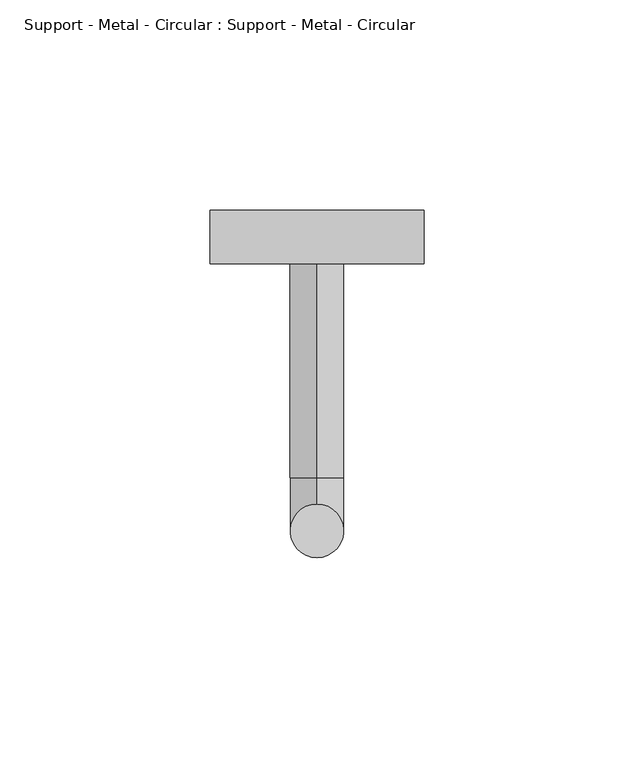
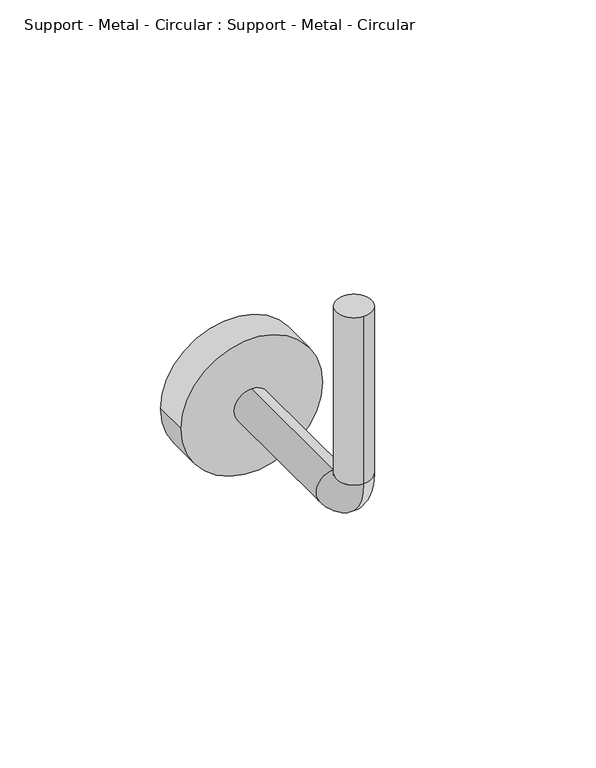
"""IFC4 building model written with IfcOpenShell, lengths in millimetres: proxy geometry, Support - Metal - Circular : Support - Metal - Circular."""

import ifcopenshell
import ifcopenshell.guid

model = None  # the IFC model being written
_history = None  # IfcOwnerHistory: only IFC2X3 demands one
_inside = {}  # id of a spatial element -> (the spatial element, [elements in it])
_under = {}  # id of a project, library or spatial element -> (it, [spatial elements below it])
_declared = {}  # id of a project -> (the project, [libraries it declares])
_typed = {}  # id of a type object -> (the type object, [elements of that type])
_made_of = {}  # id of a material, layer set ... -> (it, [elements and type objects made of it])


def new_model(schema):
    """Start an empty IFC model of exactly this schema.

    Asked for "IFC4X3", IfcOpenShell would pick the latest addendum, in which some entities
    have other attributes; the version numbers below select the first issue.
    IFC2X3 requires an IfcOwnerHistory on every rooted entity: one is made here for all.
    """
    global model, _history
    if schema == "IFC4X3":
        model = ifcopenshell.file(schema_version=(4, 3, 0, 0))
    else:
        model = ifcopenshell.file(schema=schema)
    _inside.clear()
    _under.clear()
    _declared.clear()
    _typed.clear()
    _made_of.clear()
    _history = None
    if model.schema == "IFC2X3":
        org = make("IfcOrganization", Name="unknown")
        user = make(
            "IfcPersonAndOrganization",
            ThePerson=make("IfcPerson", FamilyName="unknown"),
            TheOrganization=org,
        )
        app = make(
            "IfcApplication",
            ApplicationDeveloper=org,
            Version="unknown",
            ApplicationFullName="unknown",
            ApplicationIdentifier="unknown",
        )
        _history = make(
            "IfcOwnerHistory",
            OwningUser=user,
            OwningApplication=app,
            ChangeAction="ADDED",
            CreationDate=0,
        )
    return model


def make(cls, **values):
    """One entity of the class cls with the attributes given. An attribute that is None is left unset."""
    return model.create_entity(
        cls, **{name: value for name, value in values.items() if value is not None}
    )


def rooted(cls, **values):
    """An entity with a GlobalId (a new one), such as an element, a storey or a relation."""
    return make(cls, GlobalId=ifcopenshell.guid.new(), OwnerHistory=_history, **values)


def si_unit(unit_type, name, prefix=None):
    """IfcSIUnit, for example si_unit("LENGTHUNIT", "METRE", prefix="MILLI")."""
    return make("IfcSIUnit", UnitType=unit_type, Prefix=prefix, Name=name)


def assignment(units):
    """IfcUnitAssignment: the units of a project."""
    return None if units is None else make("IfcUnitAssignment", Units=units)


def point(xyz):
    """IfcCartesianPoint."""
    return None if xyz is None else make("IfcCartesianPoint", Coordinates=xyz)


def direction(xyz):
    """IfcDirection."""
    return None if xyz is None else make("IfcDirection", DirectionRatios=xyz)


def frame(location, z_axis=None, x_axis=None):
    """IfcAxis2Placement3D, a coordinate frame: its origin and axes. An axis left out is left unset."""
    return make(
        "IfcAxis2Placement3D",
        Location=point(location),
        Axis=direction(z_axis),
        RefDirection=direction(x_axis),
    )


def frame_2d(location, x_axis=None):
    """IfcAxis2Placement2D, a coordinate frame in the plane: its origin and x axis."""
    return make(
        "IfcAxis2Placement2D", Location=point(location), RefDirection=direction(x_axis)
    )


def origin():
    """The frame at (0, 0, 0) with its axes left unset."""
    return frame((0.0, 0.0, 0.0))


def origin_with_axes():
    """The frame at (0, 0, 0) with the z axis (0, 0, 1) and the x axis (1, 0, 0) written out."""
    return frame((0.0, 0.0, 0.0), z_axis=(0.0, 0.0, 1.0), x_axis=(1.0, 0.0, 0.0))


def place(relative_to, where):
    """IfcLocalPlacement: puts the frame where relative to a parent placement (None: the world)."""
    return make(
        "IfcLocalPlacement", PlacementRelTo=relative_to, RelativePlacement=where
    )


def context(
    kind, dimensions, precision=None, world=None, true_north=None, identifier=None
):
    """IfcGeometricRepresentationContext, for example the 3D "Model" context."""
    return make(
        "IfcGeometricRepresentationContext",
        ContextIdentifier=identifier,
        ContextType=kind,
        CoordinateSpaceDimension=dimensions,
        Precision=precision,
        WorldCoordinateSystem=world,
        TrueNorth=true_north,
    )


def project(units=None, contexts=None):
    """IfcProject with its units and contexts."""
    return rooted(
        "IfcProject",
        Name="project",
        RepresentationContexts=contexts,
        UnitsInContext=assignment(units),
    )


def spatial(cls, under=None, at=None, **own):
    """A site, building, storey or space (cls), placed at a placement, below another one or the project."""
    s = rooted(cls, ObjectPlacement=at, **own)
    if under is not None:
        _under.setdefault(under.id(), (under, []))[1].append(s)
    return s


def circle_curve(where, radius):
    """IfcCircle in the frame where."""
    return make("IfcCircle", Position=where, Radius=radius)


def ellipse_curve(where, semi_axis1, semi_axis2):
    """IfcEllipse in the frame where."""
    return make(
        "IfcEllipse", Position=where, SemiAxis1=semi_axis1, SemiAxis2=semi_axis2
    )


def trimmed(basis, trim1, trim2, sense, master):
    """IfcTrimmedCurve: the piece of a basis curve between two trims."""
    return make(
        "IfcTrimmedCurve",
        BasisCurve=basis,
        Trim1=trim1,
        Trim2=trim2,
        SenseAgreement=sense,
        MasterRepresentation=master,
    )


def segment(curve, same_sense, transition):
    """IfcCompositeCurveSegment."""
    return make(
        "IfcCompositeCurveSegment",
        Transition=transition,
        SameSense=same_sense,
        ParentCurve=curve,
    )


def composite_curve(segments, self_intersect=None):
    """IfcCompositeCurve: segments joined end to end."""
    return make("IfcCompositeCurve", Segments=segments, SelfIntersect=self_intersect)


def outline(outer, holes=None, kind="AREA"):
    """IfcArbitraryClosedProfileDef: a profile drawn as a closed curve; with holes, ...WithVoids."""
    if holes is None:
        return make("IfcArbitraryClosedProfileDef", ProfileType=kind, OuterCurve=outer)
    return make(
        "IfcArbitraryProfileDefWithVoids",
        ProfileType=kind,
        OuterCurve=outer,
        InnerCurves=holes,
    )


def extrude(swept, where, along, depth):
    """IfcExtrudedAreaSolid: the profile swept, set in the frame where, extruded along a direction by depth."""
    return make(
        "IfcExtrudedAreaSolid",
        SweptArea=swept,
        Position=where,
        ExtrudedDirection=direction(along),
        Depth=depth,
    )


def shape(context_of_items, identifier, shape_type, items):
    """IfcShapeRepresentation: the items that make up one representation, for example the "Body"."""
    return make(
        "IfcShapeRepresentation",
        ContextOfItems=context_of_items,
        RepresentationIdentifier=identifier,
        RepresentationType=shape_type,
        Items=items,
    )


def source(mapping_origin, context_of_items, identifier, shape_type, items):
    """IfcRepresentationMap: a shape defined once, which mapped items show again and again."""
    return make(
        "IfcRepresentationMap",
        MappingOrigin=mapping_origin,
        MappedRepresentation=shape(context_of_items, identifier, shape_type, items),
    )


def transform(
    local_origin,
    x_axis=None,
    y_axis=None,
    z_axis=None,
    scale=None,
    scale2=None,
    scale3=None,
    uniform=True,
):
    """IfcCartesianTransformationOperator3D, or its non-uniform kind. x_axis, y_axis, z_axis: its Axis1, 2, 3."""
    if uniform:
        return make(
            "IfcCartesianTransformationOperator3D",
            Axis1=direction(x_axis),
            Axis2=direction(y_axis),
            LocalOrigin=point(local_origin),
            Scale=scale,
            Axis3=direction(z_axis),
        )
    return make(
        "IfcCartesianTransformationOperator3DnonUniform",
        Axis1=direction(x_axis),
        Axis2=direction(y_axis),
        LocalOrigin=point(local_origin),
        Scale=scale,
        Axis3=direction(z_axis),
        Scale2=scale2,
        Scale3=scale3,
    )


def mapped(mapping_source, mapping_target):
    """IfcMappedItem: shows the shape of a source again, moved by a transform."""
    return make(
        "IfcMappedItem", MappingSource=mapping_source, MappingTarget=mapping_target
    )


def made_of(thing, what):
    """Note that an element or type object is made of a material, layer set ...; save() writes the relation."""
    if what is not None:
        _made_of.setdefault(what.id(), (what, []))[1].append(thing)
    return thing


def element(
    cls,
    number,
    at=None,
    inside=None,
    cuts=None,
    type_object=None,
    material=None,
    context=None,
    identifier="Body",
    shape_type=None,
    held_by="IfcProductDefinitionShape",
    body=None,
    shapes=None,
    **own,
):
    """One element of the class cls, such as IfcWall. Its Tag is "e" and its number.

    at: its placement. inside: the storey or other place that contains it. cuts: it is an
    opening in that element (IfcRelVoidsElement). A single representation is given by context,
    identifier, shape_type and body (its items); several are given by shapes. held_by: the class
    of the entity that holds the representations. save() writes the other relations.
    """
    e = rooted(cls, Tag="e%d" % number, ObjectPlacement=at, **own)
    if body is not None:
        shapes = [shape(context, identifier, shape_type, body)]
    if shapes is not None:
        e.Representation = make(held_by, Representations=shapes)
    if inside is not None:
        _inside.setdefault(inside.id(), (inside, []))[1].append(e)
    if cuts is not None:
        rooted(
            "IfcRelVoidsElement", RelatingBuildingElement=cuts, RelatedOpeningElement=e
        )
    if type_object is not None:
        _typed.setdefault(type_object.id(), (type_object, []))[1].append(e)
    return made_of(e, material)


def aggregate(whole, parts):
    """IfcRelAggregates: a whole, such as a stair, and the parts it consists of."""
    return rooted("IfcRelAggregates", RelatingObject=whole, RelatedObjects=parts)


def save(model, path):
    """Write the relations noted so far, then the file.

    IfcRelAggregates (storeys below a building ...), IfcRelContainedInSpatialStructure (elements
    in a storey), IfcRelDefinesByType, IfcRelAssociatesMaterial and IfcRelDeclares: one each for
    every whole, place, type object, material and project.
    """
    for whole, parts in _under.values():
        aggregate(whole, parts)
    for where, things in _inside.values():
        rooted(
            "IfcRelContainedInSpatialStructure",
            RelatedElements=things,
            RelatingStructure=where,
        )
    for kind, things in _typed.values():
        rooted("IfcRelDefinesByType", RelatedObjects=things, RelatingType=kind)
    for what, things in _made_of.values():
        rooted("IfcRelAssociatesMaterial", RelatedObjects=things, RelatingMaterial=what)
    for by, libraries in _declared.values():
        rooted("IfcRelDeclares", RelatingContext=by, RelatedDefinitions=libraries)
    model.write(path)


def plane_surface(at):
    """IfcPlane: the flat surface through the origin of the frame at, square to its z axis."""
    return make("IfcPlane", Position=at)


def cylinder_surface(at, radius):
    """IfcCylindricalSurface: all points at the distance radius from the z axis of the frame at."""
    return make("IfcCylindricalSurface", Position=at, Radius=radius)


def revolved_surface(curve, axis_point, axis_direction):
    """IfcSurfaceOfRevolution: the curve turned about the line through axis_point along axis_direction."""
    return make(
        "IfcSurfaceOfRevolution",
        SweptCurve=make("IfcArbitraryOpenProfileDef", ProfileType="CURVE", Curve=curve),
        AxisPosition=make("IfcAxis1Placement", Location=point(axis_point), Axis=direction(axis_direction)),
    )


def advanced_brep(points, edges, surfaces, faces):
    """IfcAdvancedBrep: a solid bounded by faces that lie on surfaces and meet in shared edges.

    An edge is (start, end): straight between two places in points (the first is 0);
    or (start, end, curve); or (start, end, curve, False) where it runs against its curve.
    A face is (place in surfaces, loops), or (place, loops, False) where it looks against
    its surface's normal. A loop lists edges by number (the first is 1), with a minus sign
    where the edge is run from its end to its start. The first loop is the outer one.
    """
    corners = [point(p) for p in points]
    vertices = [make("IfcVertexPoint", VertexGeometry=c) for c in corners]
    made = []
    for start, end, *more in edges:
        made.append(
            make(
                "IfcEdgeCurve",
                EdgeStart=vertices[start],
                EdgeEnd=vertices[end],
                EdgeGeometry=more[0] if more else make("IfcPolyline", Points=[corners[start], corners[end]]),
                SameSense=more[1] if len(more) > 1 else True,
            )
        )
    hull = []
    for where, loops, *sense in faces:
        bounds = []
        for j, loop in enumerate(loops):
            ring = [make("IfcOrientedEdge", EdgeElement=made[abs(k) - 1], Orientation=k > 0) for k in loop]
            bounds.append(
                make(
                    "IfcFaceOuterBound" if j == 0 else "IfcFaceBound",
                    Bound=make("IfcEdgeLoop", EdgeList=ring),
                    Orientation=True,
                )
            )
        hull.append(make("IfcAdvancedFace", Bounds=bounds, FaceSurface=surfaces[where], SameSense=sense[0] if sense else True))
    return make("IfcAdvancedBrep", Outer=make("IfcClosedShell", CfsFaces=hull))


def support_metal_circular_support_metal_circular_6fb01533(model_context):
    return source(origin(), model_context, "Body", "SolidModel", [
        advanced_brep(
        [(0.0, 63.5, -69.85), (0.0, 63.5, -82.55), (0.0, 12.7, -69.85), (0.0, 12.7, -82.55), (0.0, -6.35, -63.5), (0.0, 6.35, -63.5), (0.0, 6.35, 0.0), (0.0, -6.35, 0.0)],
        [
            (0, 1, circle_curve(frame((0.0, 63.5, -76.2), z_axis=(0.0, 1.0, 0.0), x_axis=(0.0, 0.0, -1.0)), 6.35)),
            (1, 0, circle_curve(frame((0.0, 63.5, -76.2), z_axis=(0.0, 1.0, 0.0), x_axis=(0.0, 0.0, -1.0)), 6.35)),
            (0, 2),
            (2, 3, circle_curve(frame((0.0, 12.7, -76.2), z_axis=(0.0, 1.0, 0.0), x_axis=(0.0, 0.0, -1.0)), 6.35)),
            (3, 1),
            (3, 2, circle_curve(frame((0.0, 12.7, -76.2), z_axis=(0.0, 1.0, 0.0), x_axis=(0.0, 0.0, -1.0)), 6.35)),
            (4, 3, circle_curve(frame((0.0, 12.7, -63.5), z_axis=(1.0, 0.0, 0.0), x_axis=(0.0, 0.0, -1.0)), 19.05)),
            (2, 5, circle_curve(frame((0.0, 12.7, -63.5), z_axis=(-1.0, 0.0, 0.0), x_axis=(0.0, 0.0, -1.0)), 6.35)),
            (5, 4, circle_curve(frame((0.0, 0.0, -63.5), z_axis=(0.0, 0.0, -1.0), x_axis=(0.0, -1.0, 0.0)), 6.35)),
            (4, 5, circle_curve(frame((0.0, 0.0, -63.5), z_axis=(0.0, 0.0, -1.0), x_axis=(0.0, -1.0, 0.0)), 6.35)),
            (6, 7, circle_curve(frame((0.0, 0.0, 0.0), z_axis=(0.0, 0.0, 1.0), x_axis=(0.0, -1.0, 0.0)), 6.35)),
            (7, 6, circle_curve(frame((0.0, 0.0, 0.0), z_axis=(0.0, 0.0, 1.0), x_axis=(0.0, -1.0, 0.0)), 6.35)),
            (5, 6),
            (7, 4),
        ],
        [
            plane_surface(frame((0.0, 63.5, -76.2), z_axis=(0.0, 1.0, 0.0), x_axis=(1.0, 0.0, 0.0))),
            cylinder_surface(frame((0.0, 63.5, -76.2), z_axis=(0.0, 1.0, 0.0), x_axis=(0.0, 0.0, -1.0)), 6.35),
            revolved_surface(trimmed(ellipse_curve(frame((0.0, 12.7, -76.2), z_axis=(0.0, 1.0, 0.0), x_axis=(0.0, 0.0, -1.0)), 6.35, 6.35), [point((0.0, 12.7, -69.85))], [point((0.0, 12.7, -82.55))], True, "CARTESIAN"), (0.0, 12.7, -63.5), (-1.0, 0.0, 0.0)),
            revolved_surface(trimmed(ellipse_curve(frame((0.0, 12.7, -76.2), z_axis=(0.0, 1.0, 0.0), x_axis=(0.0, 0.0, -1.0)), 6.35, 6.35), [point((0.0, 12.7, -82.55))], [point((0.0, 12.7, -69.85))], True, "CARTESIAN"), (0.0, 12.7, -63.5), (-1.0, 0.0, 0.0)),
            plane_surface(origin_with_axes()),
            cylinder_surface(frame((0.0, 0.0, -63.5), z_axis=(0.0, 0.0, -1.0), x_axis=(0.0, -1.0, 0.0)), 6.35),
        ],
        [
            (0, [[1, 2]]),
            (1, [[-1, 3, 4, 5]]),
            (1, [[-2, -5, 6, -3]]),
            (2, [[7, -4, 8, 9]]),
            (3, [[-8, -6, -7, 10]]),
            (4, [[11, 12]]),
            (5, [[-9, 13, -12, 14]]),
            (5, [[-10, -14, -11, -13]]),
        ],
    ),
        extrude(outline(composite_curve([segment(trimmed(circle_curve(frame_2d((-76.2, 0.0)), 25.4), [point((-76.2, -25.4))], [point((-76.2, 25.4))], False, "CARTESIAN"), True, "CONTINUOUS"), segment(trimmed(circle_curve(frame_2d((-76.2, 0.0)), 25.4), [point((-76.2, 25.4))], [point((-76.2, -25.4))], False, "CARTESIAN"), True, "CONTINUOUS")], self_intersect=False)), frame((0.0, 63.5, 0.0), z_axis=(0.0, 1.0, 0.0), x_axis=(0.0, 0.0, 1.0)), (0.0, 0.0, 1.0), 12.7),
    ])


if __name__ == "__main__":
    model = new_model("IFC4")
    model_context = context("Model", 3, world=origin())
    ifc_project = project(units=[si_unit("LENGTHUNIT", "METRE", prefix="MILLI")], contexts=[model_context])
    site = spatial("IfcSite", under=ifc_project)
    building = spatial("IfcBuilding", under=site)
    placement = place(None, origin())
    support_metal_circular_support_metal_circular_shape = support_metal_circular_support_metal_circular_6fb01533(model_context)
    element("IfcBuildingElementProxy", 1, Name="Support - Metal - Circular : Support - Metal - Circular", ObjectType="Support - Metal - Circular : Support - Metal - Circular", at=placement, inside=building, context=model_context, shape_type="MappedRepresentation", body=[
        mapped(support_metal_circular_support_metal_circular_shape, transform((0.0, 0.0, 0.0), x_axis=(1.0, 0.0, 0.0), y_axis=(0.0, 1.0, 0.0), z_axis=(0.0, 0.0, 1.0))),
    ])
    save(model, "model.ifc")

# Revit data of these elements
# Type "Support - Metal - Circular : Support - Metal - Circular"
#   T1 = 0' - 0 1/2"
#   Radius 1 = 0' - 1"
#   Radius 2 = 0' - 0 1/4"
#   built-in parameter 1152166 = 0.25 (stored number, unit not read)
#   built-in parameter 1152165 [instance default] = 0.25 (stored number, unit not read)
#   Bend Radius = 0' - 0 1/2"
#   Support Material = Aluminum
# Element 1 (IfcBuildingElementProxy, "Support - Metal - Circular : Support - Metal - Circular")
#   Materials on its faces: "Aluminum"
# Materials
#   "Aluminum": class "Metal", colour RGB 247 247 247, transparency 0, Description = "Aluminum 6061", Cost = 0
